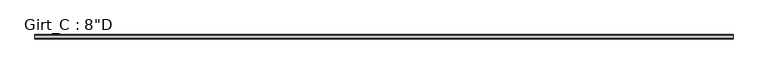
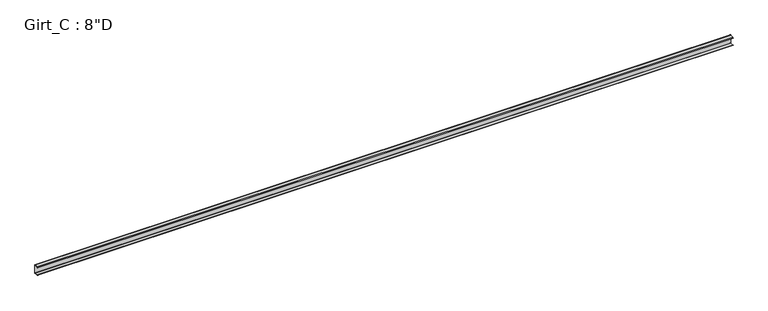
"""IFC4 building model written with IfcOpenShell, lengths in millimetres: beam geometry."""

from ifc_helpers import new_model, si_unit, point, frame, frame_2d, origin, place, context, project, spatial, polyline, circle_curve, trimmed, segment, composite_curve, outline, extrude, source, transform, mapped, element, save


def beam_6849cdf3(model_context):
    return source(origin(), model_context, "Body", "SweptSolid", [
        extrude(outline(composite_curve([segment(polyline([(-87.5109375, 101.6), (-3.3734375, 101.6)]), True, "CONTINUOUS"), segment(trimmed(circle_curve(frame_2d((-3.3734375, 96.8375)), 4.7625), [point((-3.3734375, 101.6))], [point((1.3890625, 96.8375))], False, "CARTESIAN"), True, "CONTINUOUS"), segment(polyline([(1.3890625, 96.8375), (1.3890625, -96.8375)]), True, "CONTINUOUS"), segment(trimmed(circle_curve(frame_2d((-3.3734375, -96.8375)), 4.7625), [point((1.3890625, -96.8375))], [point((-3.3734375, -101.6))], False, "CARTESIAN"), True, "CONTINUOUS"), segment(polyline([(-3.3734375, -101.6), (-87.5109375, -101.6), (-99.7792647, -86.979177), (-97.6510975, -85.1934327), (-86.2154765, -98.821875), (-3.2694106, -98.821875)]), True, "CONTINUOUS"), segment(trimmed(circle_curve(frame_2d((-3.3748024, -96.8389339)), 1.9857399), [point((-3.2694106, -98.821875))], [point((-1.3890625, -96.8389339))], True, "CARTESIAN"), True, "CONTINUOUS"), segment(polyline([(-1.3890625, -96.8389339), (-1.3890625, 96.8381931)]), True, "CONTINUOUS"), segment(trimmed(circle_curve(frame_2d((-3.3741066, 96.8381931)), 1.9850441), [point((-1.3890625, 96.8381931))], [point((-3.3005807, 98.821875))], True, "CARTESIAN"), True, "CONTINUOUS"), segment(polyline([(-3.3005807, 98.821875), (-86.2154765, 98.821875), (-97.6278742, 85.221109), (-99.7560415, 87.0068534), (-87.5109375, 101.6)]), True, "CONTINUOUS")], self_intersect=False)), frame((-8066.3936327, 0.0, 0.0), z_axis=(1.0, 0.0, 0.0), x_axis=(0.0, 1.0, 0.0)), (0.0, 0.0, 1.0), 16036.6954874),
    ])


if __name__ == "__main__":
    model = new_model("IFC4")
    model_context = context("Model", 3, world=origin())
    ifc_project = project(units=[si_unit("LENGTHUNIT", "METRE", prefix="MILLI")], contexts=[model_context])
    site = spatial("IfcSite", under=ifc_project)
    building = spatial("IfcBuilding", under=site)
    placement = place(None, origin())
    beam_shape = beam_6849cdf3(model_context)
    element("IfcBeam", 1, ObjectType="Girt_C : 8\"D", at=placement, inside=building, context=model_context, shape_type="MappedRepresentation", body=[
        mapped(beam_shape, transform((0.0, 0.0, 0.0), x_axis=(1.0, 0.0, 0.0), y_axis=(0.0, 1.0, 0.0), z_axis=(0.0, 0.0, 1.0))),
    ])
    save(model, "model.ifc")

# Revit data of these elements
# Type "Girt_C : 8\"D"
#   half leg = 0' - 1 3/4"
#   Web_Thickness = 0' - 0 7/64"
#   Length [instance default] = 10' - 0"
#   Leg_1 = 0' - 3 1/2"
#   Height = 0' - 8"
#   Structural Material [instance default] = none
# Element 1 (IfcBeam, "Girt_C : 8\"D")
#   Structural Material = GALVANIZED 'CEE' SECTION (8.0x3.5C - SEE STRUCT. DWGS)
#   Materials on its faces: "GALVANIZED 'CEE' SECTION (8.0x3.5C - SEE STRUCT. DWGS)"
# Materials
#   "GALVANIZED 'CEE' SECTION (8.0x3.5C - SEE STRUCT. DWGS)": class "Metal", colour RGB 137 146 153, transparency 0, Description = "Steel, mill finish", Cost = 0
